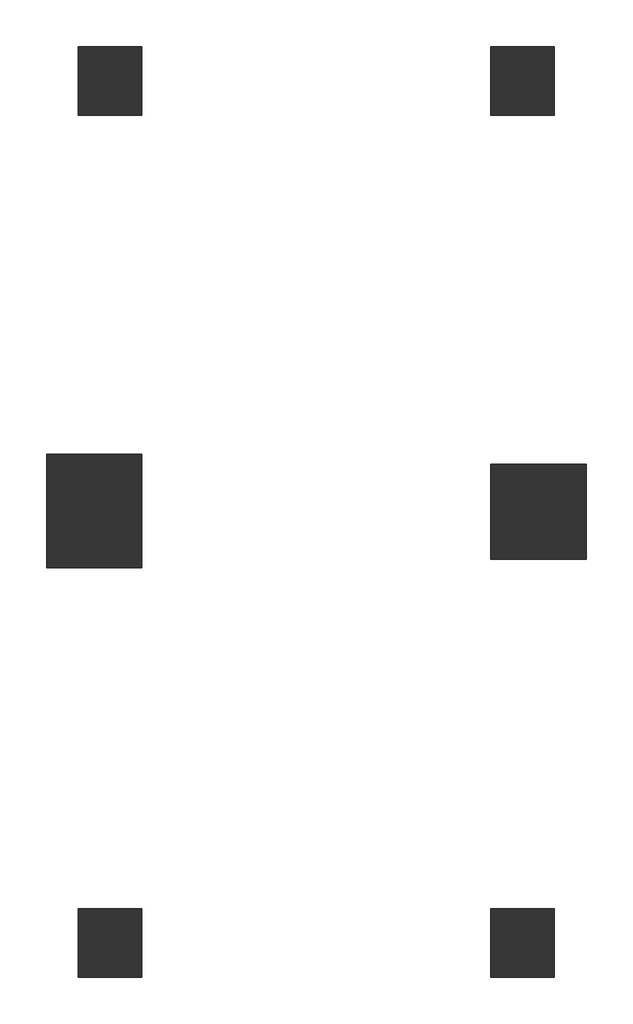
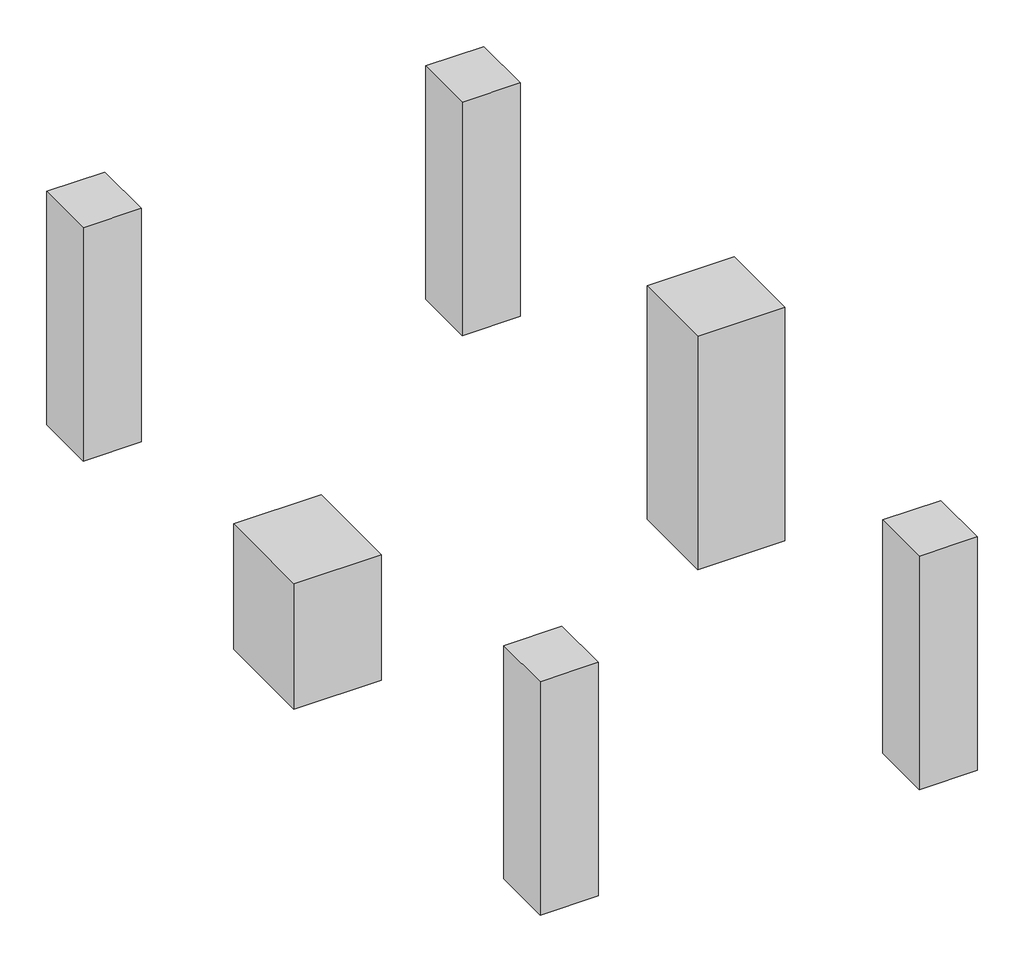
# One storey: 6 columns.
"""IFC4 building model written with IfcOpenShell, lengths in millimetres."""

import ifcopenshell
import ifcopenshell.guid

model = None  # the IFC model being written
_history = None  # IfcOwnerHistory: only IFC2X3 demands one
_inside = {}  # id of a spatial element -> (the spatial element, [elements in it])
_under = {}  # id of a project, library or spatial element -> (it, [spatial elements below it])
_declared = {}  # id of a project -> (the project, [libraries it declares])
_typed = {}  # id of a type object -> (the type object, [elements of that type])
_made_of = {}  # id of a material, layer set ... -> (it, [elements and type objects made of it])


def new_model(schema):
    """Start an empty IFC model of exactly this schema.

    Asked for "IFC4X3", IfcOpenShell would pick the latest addendum, in which some entities
    have other attributes; the version numbers below select the first issue.
    IFC2X3 requires an IfcOwnerHistory on every rooted entity: one is made here for all.
    """
    global model, _history
    if schema == "IFC4X3":
        model = ifcopenshell.file(schema_version=(4, 3, 0, 0))
    else:
        model = ifcopenshell.file(schema=schema)
    _inside.clear()
    _under.clear()
    _declared.clear()
    _typed.clear()
    _made_of.clear()
    _history = None
    if model.schema == "IFC2X3":
        org = make("IfcOrganization", Name="unknown")
        user = make(
            "IfcPersonAndOrganization",
            ThePerson=make("IfcPerson", FamilyName="unknown"),
            TheOrganization=org,
        )
        app = make(
            "IfcApplication",
            ApplicationDeveloper=org,
            Version="unknown",
            ApplicationFullName="unknown",
            ApplicationIdentifier="unknown",
        )
        _history = make(
            "IfcOwnerHistory",
            OwningUser=user,
            OwningApplication=app,
            ChangeAction="ADDED",
            CreationDate=0,
        )
    return model


def make(cls, **values):
    """One entity of the class cls with the attributes given. An attribute that is None is left unset."""
    return model.create_entity(
        cls, **{name: value for name, value in values.items() if value is not None}
    )


def rooted(cls, **values):
    """An entity with a GlobalId (a new one), such as an element, a storey or a relation."""
    return make(cls, GlobalId=ifcopenshell.guid.new(), OwnerHistory=_history, **values)


def si_unit(unit_type, name, prefix=None):
    """IfcSIUnit, for example si_unit("LENGTHUNIT", "METRE", prefix="MILLI")."""
    return make("IfcSIUnit", UnitType=unit_type, Prefix=prefix, Name=name)


def assignment(units):
    """IfcUnitAssignment: the units of a project."""
    return None if units is None else make("IfcUnitAssignment", Units=units)


def point(xyz):
    """IfcCartesianPoint."""
    return None if xyz is None else make("IfcCartesianPoint", Coordinates=xyz)


def direction(xyz):
    """IfcDirection."""
    return None if xyz is None else make("IfcDirection", DirectionRatios=xyz)


def frame(location, z_axis=None, x_axis=None):
    """IfcAxis2Placement3D, a coordinate frame: its origin and axes. An axis left out is left unset."""
    return make(
        "IfcAxis2Placement3D",
        Location=point(location),
        Axis=direction(z_axis),
        RefDirection=direction(x_axis),
    )


def origin():
    """The frame at (0, 0, 0) with its axes left unset."""
    return frame((0.0, 0.0, 0.0))


def place(relative_to, where):
    """IfcLocalPlacement: puts the frame where relative to a parent placement (None: the world)."""
    return make(
        "IfcLocalPlacement", PlacementRelTo=relative_to, RelativePlacement=where
    )


def context(
    kind, dimensions, precision=None, world=None, true_north=None, identifier=None
):
    """IfcGeometricRepresentationContext, for example the 3D "Model" context."""
    return make(
        "IfcGeometricRepresentationContext",
        ContextIdentifier=identifier,
        ContextType=kind,
        CoordinateSpaceDimension=dimensions,
        Precision=precision,
        WorldCoordinateSystem=world,
        TrueNorth=true_north,
    )


def project(units=None, contexts=None):
    """IfcProject with its units and contexts."""
    return rooted(
        "IfcProject",
        Name="project",
        RepresentationContexts=contexts,
        UnitsInContext=assignment(units),
    )


def spatial(cls, under=None, at=None, **own):
    """A site, building, storey or space (cls), placed at a placement, below another one or the project."""
    s = rooted(cls, ObjectPlacement=at, **own)
    if under is not None:
        _under.setdefault(under.id(), (under, []))[1].append(s)
    return s


def polyline(points):
    """IfcPolyline through the points."""
    return make("IfcPolyline", Points=[point(p) for p in points])


def outline(outer, holes=None, kind="AREA"):
    """IfcArbitraryClosedProfileDef: a profile drawn as a closed curve; with holes, ...WithVoids."""
    if holes is None:
        return make("IfcArbitraryClosedProfileDef", ProfileType=kind, OuterCurve=outer)
    return make(
        "IfcArbitraryProfileDefWithVoids",
        ProfileType=kind,
        OuterCurve=outer,
        InnerCurves=holes,
    )


def extrude(swept, where, along, depth):
    """IfcExtrudedAreaSolid: the profile swept, set in the frame where, extruded along a direction by depth."""
    return make(
        "IfcExtrudedAreaSolid",
        SweptArea=swept,
        Position=where,
        ExtrudedDirection=direction(along),
        Depth=depth,
    )


def shape(context_of_items, identifier, shape_type, items):
    """IfcShapeRepresentation: the items that make up one representation, for example the "Body"."""
    return make(
        "IfcShapeRepresentation",
        ContextOfItems=context_of_items,
        RepresentationIdentifier=identifier,
        RepresentationType=shape_type,
        Items=items,
    )


def source(mapping_origin, context_of_items, identifier, shape_type, items):
    """IfcRepresentationMap: a shape defined once, which mapped items show again and again."""
    return make(
        "IfcRepresentationMap",
        MappingOrigin=mapping_origin,
        MappedRepresentation=shape(context_of_items, identifier, shape_type, items),
    )


def transform(
    local_origin,
    x_axis=None,
    y_axis=None,
    z_axis=None,
    scale=None,
    scale2=None,
    scale3=None,
    uniform=True,
):
    """IfcCartesianTransformationOperator3D, or its non-uniform kind. x_axis, y_axis, z_axis: its Axis1, 2, 3."""
    if uniform:
        return make(
            "IfcCartesianTransformationOperator3D",
            Axis1=direction(x_axis),
            Axis2=direction(y_axis),
            LocalOrigin=point(local_origin),
            Scale=scale,
            Axis3=direction(z_axis),
        )
    return make(
        "IfcCartesianTransformationOperator3DnonUniform",
        Axis1=direction(x_axis),
        Axis2=direction(y_axis),
        LocalOrigin=point(local_origin),
        Scale=scale,
        Axis3=direction(z_axis),
        Scale2=scale2,
        Scale3=scale3,
    )


def mapped(mapping_source, mapping_target):
    """IfcMappedItem: shows the shape of a source again, moved by a transform."""
    return make(
        "IfcMappedItem", MappingSource=mapping_source, MappingTarget=mapping_target
    )


def made_of(thing, what):
    """Note that an element or type object is made of a material, layer set ...; save() writes the relation."""
    if what is not None:
        _made_of.setdefault(what.id(), (what, []))[1].append(thing)
    return thing


def element(
    cls,
    number,
    at=None,
    inside=None,
    cuts=None,
    type_object=None,
    material=None,
    context=None,
    identifier="Body",
    shape_type=None,
    held_by="IfcProductDefinitionShape",
    body=None,
    shapes=None,
    **own,
):
    """One element of the class cls, such as IfcWall. Its Tag is "e" and its number.

    at: its placement. inside: the storey or other place that contains it. cuts: it is an
    opening in that element (IfcRelVoidsElement). A single representation is given by context,
    identifier, shape_type and body (its items); several are given by shapes. held_by: the class
    of the entity that holds the representations. save() writes the other relations.
    """
    e = rooted(cls, Tag="e%d" % number, ObjectPlacement=at, **own)
    if body is not None:
        shapes = [shape(context, identifier, shape_type, body)]
    if shapes is not None:
        e.Representation = make(held_by, Representations=shapes)
    if inside is not None:
        _inside.setdefault(inside.id(), (inside, []))[1].append(e)
    if cuts is not None:
        rooted(
            "IfcRelVoidsElement", RelatingBuildingElement=cuts, RelatedOpeningElement=e
        )
    if type_object is not None:
        _typed.setdefault(type_object.id(), (type_object, []))[1].append(e)
    return made_of(e, material)


def aggregate(whole, parts):
    """IfcRelAggregates: a whole, such as a stair, and the parts it consists of."""
    return rooted("IfcRelAggregates", RelatingObject=whole, RelatedObjects=parts)


def save(model, path):
    """Write the relations noted so far, then the file.

    IfcRelAggregates (storeys below a building ...), IfcRelContainedInSpatialStructure (elements
    in a storey), IfcRelDefinesByType, IfcRelAssociatesMaterial and IfcRelDeclares: one each for
    every whole, place, type object, material and project.
    """
    for whole, parts in _under.values():
        aggregate(whole, parts)
    for where, things in _inside.values():
        rooted(
            "IfcRelContainedInSpatialStructure",
            RelatedElements=things,
            RelatingStructure=where,
        )
    for kind, things in _typed.values():
        rooted("IfcRelDefinesByType", RelatedObjects=things, RelatingType=kind)
    for what, things in _made_of.values():
        rooted("IfcRelAssociatesMaterial", RelatedObjects=things, RelatingMaterial=what)
    for by, libraries in _declared.values():
        rooted("IfcRelDeclares", RelatingContext=by, RelatedDefinitions=libraries)
    model.write(path)


def rc_column_rectangular_f1dd4ac0(model_context):
    return source(origin(), model_context, "Body", "SweptSolid", [
        extrude(outline(polyline([(300.0, 325.0), (300.0, -325.0), (-300.0, -325.0), (-300.0, 325.0), (300.0, 325.0)])), frame((0.0, 0.0, 4799.9618634), z_axis=(0.0, 0.0, 1.0), x_axis=(1.0, 0.0, 0.0)), (0.0, 0.0, 1.0), 2540.0381366),
    ])


def rc_column_rectangular_84820dcc(model_context):
    return source(origin(), model_context, "Body", "SweptSolid", [
        extrude(outline(polyline([(450.0, 450.0), (450.0, -450.0), (-450.0, -450.0), (-450.0, 450.0), (450.0, 450.0)])), frame((0.0, 0.0, 4799.9618634), z_axis=(0.0, 0.0, 1.0), x_axis=(1.0, 0.0, 0.0)), (0.0, 0.0, 1.0), 2540.0381366),
    ])


def rc_column_rectangular_1dd1414b(model_context):
    return source(origin(), model_context, "Body", "SweptSolid", [
        extrude(outline(polyline([(450.0, 535.0), (450.0, -535.0), (-450.0, -535.0), (-450.0, 535.0), (450.0, 535.0)])), frame((0.0, 0.0, 4799.9618634), z_axis=(0.0, 0.0, 1.0), x_axis=(1.0, 0.0, 0.0)), (0.0, 0.0, 1.0), 1365.0381366),
    ])


model = new_model("IFC4")

# Units and contexts
model_context = context("Model", 3, world=origin())
ifc_project = project(units=[si_unit("LENGTHUNIT", "METRE", prefix="MILLI")], contexts=[model_context])

# Site, building, storey
site = spatial("IfcSite", under=ifc_project)
building = spatial("IfcBuilding", under=site)
storey = spatial("IfcBuildingStorey", under=building, Name="T.O.C", Elevation=4799.9618634)

# Columns
placement = place(None, origin())
rc_column_rectangular_shape = rc_column_rectangular_f1dd4ac0(model_context)
element("IfcColumn", 1, ObjectType="RC_Column_Rectangular : H_SC_AR_S15_AG Column_600x650_C3", at=placement, inside=storey, context=model_context, shape_type="MappedRepresentation", body=[
    mapped(rc_column_rectangular_shape, transform((20010.0, -7764.2216244, 0.0), x_axis=(1.0, 0.0, 0.0), y_axis=(0.0, 1.0, 0.0), z_axis=(0.0, 0.0, 1.0))),
])
element("IfcColumn", 2, ObjectType="RC_Column_Rectangular : H_SC_AR_S15_AG Column_600x650_C3", at=placement, inside=storey, context=model_context, shape_type="MappedRepresentation", body=[
    mapped(rc_column_rectangular_shape, transform((23910.0, -7764.2216244, 0.0), x_axis=(1.0, 0.0, 0.0), y_axis=(0.0, 1.0, 0.0), z_axis=(0.0, 0.0, 1.0))),
])
element("IfcColumn", 3, ObjectType="RC_Column_Rectangular : H_SC_AR_S15_AG Column_600x650_C3", at=placement, inside=storey, context=model_context, shape_type="MappedRepresentation", body=[
    mapped(rc_column_rectangular_shape, transform((20010.0, -15911.5096992, 0.0), x_axis=(1.0, 0.0, 0.0), y_axis=(0.0, 1.0, 0.0), z_axis=(0.0, 0.0, 1.0))),
])
element("IfcColumn", 4, ObjectType="RC_Column_Rectangular : H_SC_AR_S15_AG Column_600x650_C3", at=placement, inside=storey, context=model_context, shape_type="MappedRepresentation", body=[
    mapped(rc_column_rectangular_shape, transform((23910.0, -15911.5096992, 0.0), x_axis=(1.0, 0.0, 0.0), y_axis=(0.0, 1.0, 0.0), z_axis=(0.0, 0.0, 1.0))),
])
rc_column_rectangular_2_shape = rc_column_rectangular_84820dcc(model_context)
element("IfcColumn", 5, ObjectType="RC_Column_Rectangular : H_SC_AR_S15_AG Column_900x900_C2", at=placement, inside=storey, context=model_context, shape_type="MappedRepresentation", body=[
    mapped(rc_column_rectangular_2_shape, transform((24060.0, -11836.5096992, 0.0), x_axis=(1.0, 0.0, 0.0), y_axis=(0.0, 1.0, 0.0), z_axis=(0.0, 0.0, 1.0))),
])
rc_column_rectangular_3_shape = rc_column_rectangular_1dd1414b(model_context)
element("IfcColumn", 6, ObjectType="RC_Column_Rectangular : H_SC_AR_S15_AG Column_900x1070_C1", at=placement, inside=storey, context=model_context, shape_type="MappedRepresentation", body=[
    mapped(rc_column_rectangular_3_shape, transform((19860.0, -11828.7667086, 0.0), x_axis=(1.0, 0.0, 0.0), y_axis=(0.0, 1.0, 0.0), z_axis=(0.0, 0.0, 1.0))),
])

save(model, "model.ifc")

# Revit data of these elements
# Type "RC_Column_Rectangular : H_SC_AR_S15_AG Column_600x650_C3"
#   Width = 600 mm
#   Length = 650 mm
#   hec_material3 [instance default] = none
#   hec_material2 [instance default] = none
#   hec_material1 [instance default] = none
#   Structural Material [instance default] = none
#   Description = (empty or 0)
# Type "RC_Column_Rectangular : H_SC_AR_S15_AG Column_900x900_C2"
#   Width = 900 mm
#   Length = 900 mm
#   hec_material3 [instance default] = none
#   hec_material2 [instance default] = none
#   hec_material1 [instance default] = none
#   Structural Material [instance default] = none
#   Description = (empty or 0)
# Type "RC_Column_Rectangular : H_SC_AR_S15_AG Column_900x1070_C1"
#   Type Comments = "CV-AG"
#   Type Mark = ""
#   Width = 900 mm
#   Length = 1070 mm
#   hec_material3 [instance default] = none
#   hec_material2 [instance default] = none
#   hec_material1 [instance default] = none
#   Structural Material [instance default] = none
#   Description = (empty or 0)
# Elements 1, 2, 3, 4 (IfcColumn, "RC_Column_Rectangular : H_SC_AR_S15_AG Column_600x650_C3")
#   Comments = ""
#   Structural Material = Concrete_f'c=28MPa(Cylender)
#   hec_material3 = none
#   hec_material2 = none
#   hec_material1 = none
#   Phase Created = New Construction
#   Materials on its faces: "Concrete_f'c=28MPa(Cylender)"
# Element 5 (IfcColumn, "RC_Column_Rectangular : H_SC_AR_S15_AG Column_900x900_C2")
#   Comments = ""
#   Structural Material = Concrete_f'c=28MPa(Cylender)
#   hec_material3 = none
#   hec_material2 = none
#   hec_material1 = none
#   Phase Created = New Construction
#   Materials on its faces: "Concrete_f'c=28MPa(Cylender)"
# Element 6 (IfcColumn, "RC_Column_Rectangular : H_SC_AR_S15_AG Column_900x1070_C1")
#   Comments = ""
#   Structural Material = Concrete_f'c=28MPa(Cylender)
#   hec_material3 = none
#   hec_material2 = none
#   hec_material1 = none
#   Phase Created = New Construction
#   Materials on its faces: "Concrete_f'c=28MPa(Cylender)"
# Materials
#   "Concrete_f'c=28MPa(Cylender)": class "Concrete", colour RGB 176 176 176, transparency 0, Description = "Reinf. Conc.", Cost = 0, Image = Concrete.Cast-In-Place.Flat.Polished.Grey.jpg
